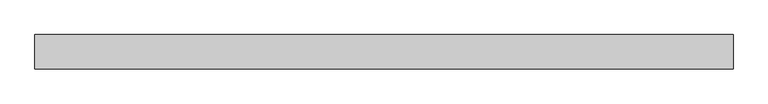
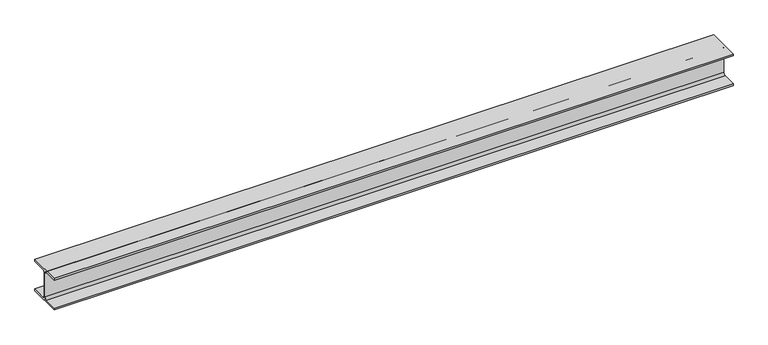
"""IFC4 building model written with IfcOpenShell, lengths in millimetres: beam geometry, 0912_Steel Framing_H-KSD3502 : H_SB_ASB_H-200x200x8x12."""

from ifc_helpers import new_model, si_unit, point, frame, frame_2d, origin, place, context, project, spatial, polyline, circle_curve, trimmed, segment, composite_curve, outline, extrude, source, transform, mapped, element, save


def beam_d7917815(model_context):
    return source(origin(), model_context, "Body", "SweptSolid", [
        extrude(outline(composite_curve([segment(polyline([(100.0, -88.0), (100.0, -100.0), (-100.0, -100.0), (-100.0, -88.0), (-17.0, -88.0)]), True, "CONTINUOUS"), segment(trimmed(circle_curve(frame_2d((-17.0, -75.0)), 13.0), [point((-17.0, -88.0))], [point((-4.0, -75.0))], True, "CARTESIAN"), True, "CONTINUOUS"), segment(polyline([(-4.0, -75.0), (-4.0, 75.0)]), True, "CONTINUOUS"), segment(trimmed(circle_curve(frame_2d((-17.0, 75.0)), 13.0), [point((-4.0, 75.0))], [point((-17.0, 88.0))], True, "CARTESIAN"), True, "CONTINUOUS"), segment(polyline([(-17.0, 88.0), (-100.0, 88.0), (-100.0, 100.0), (100.0, 100.0), (100.0, 88.0), (17.0, 88.0)]), True, "CONTINUOUS"), segment(trimmed(circle_curve(frame_2d((17.0, 75.0)), 13.0), [point((17.0, 88.0))], [point((4.0, 75.0))], True, "CARTESIAN"), True, "CONTINUOUS"), segment(polyline([(4.0, 75.0), (4.0, -75.0)]), True, "CONTINUOUS"), segment(trimmed(circle_curve(frame_2d((17.0, -75.0)), 13.0), [point((4.0, -75.0))], [point((17.0, -88.0))], True, "CARTESIAN"), True, "CONTINUOUS"), segment(polyline([(17.0, -88.0), (100.0, -88.0)]), True, "CONTINUOUS")], self_intersect=False)), frame((-2035.0333333, 0.0, 0.0), z_axis=(1.0, 0.0, 0.0), x_axis=(0.0, 1.0, 0.0)), (0.0, 0.0, 1.0), 4070.0666667),
    ])


if __name__ == "__main__":
    model = new_model("IFC4")
    model_context = context("Model", 3, world=origin())
    ifc_project = project(units=[si_unit("LENGTHUNIT", "METRE", prefix="MILLI")], contexts=[model_context])
    site = spatial("IfcSite", under=ifc_project)
    building = spatial("IfcBuilding", under=site)
    placement = place(None, origin())
    beam_shape = beam_d7917815(model_context)
    element("IfcBeam", 1, ObjectType="0912_Steel Framing_H-KSD3502 : H_SB_ASB_H-200x200x8x12", at=placement, inside=building, context=model_context, shape_type="MappedRepresentation", body=[
        mapped(beam_shape, transform((0.0, 0.0, 0.0), x_axis=(1.0, 0.0, 0.0), y_axis=(0.0, 1.0, 0.0), z_axis=(0.0, 0.0, 1.0))),
    ])
    save(model, "model.ifc")

# Revit data of these elements
# Type "0912_Steel Framing_H-KSD3502 : H_SB_ASB_H-200x200x8x12"
#   H_WM Code_1 = "S01AA002-00001 | Main Steel Structure Fabrication Work | Shelter/Building | Medium Steel - Standard (90KG/M>Weight≥30KG/M) | Material: (   )"
#   H_WM Code_2 = "S03AA028-00001 | Main Steel Structure Erection Work | Shelter/Building | Medium Steel (90KG/M>Weight≥30KG/M) | Material: (   )"
#   H_WM Code_3 = "S01AA010-00001 | Main Steel Structure Fabrication Work | Shelter/Building | Steel Painting/Coating | for Non-Fireproofed Steel Surface, Surface Preparation, Primer, Second & Final Coat | Material: (   )"
#   H_Q'ty Cal Type Tag = "SB-Q2"
#   Width = 20.0 cm
#   Web Thickness = 0.8 cm
#   Web Fillet = 1.3 cm
#   Warping Constant = 141000.0 cm⁶
#   W = 0
#   Torsional Moment of Inertia = 26.2485 cm⁴
#   Section Area = 63.53 cm²
#   Plastic Modulus weak axis = 244.0 cm³
#   Plastic Modulus strong axis = 525.0 cm³
#   Perimeter = 1.16 m²/m
#   Nominal Weight = 49.90 kgf/m
#   Moment of Inertia weak axis = 1600.00 cm⁴
#   Moment of Inertia strong axis = 4720.00 cm⁴
#   Height = 20.0 cm
#   Flange Thickness = 1.2 cm
#   Elastic Modulus weak axis = 160.0 cm³
#   Elastic Modulus strong axis = 472.0 cm³
#   Centroid Vertical = 10.0 cm
#   Centroid Horizontal = 10.0 cm
#   Ix = 47200000
#   Length [instance default] = 1.5240 m
#   Zx = 525000
#   b = 0.2000 m
#   h = 0.2000 m
#   r = 0.0130 m
#   s = 0.0080 m
#   t = 0.0120 m
#   A = 0.006353 m²
#   Structural Material [instance default] = Steel, 45-345
#   Assembly Code = ""
# Element 1 (IfcBeam, "0912_Steel Framing_H-KSD3502 : H_SB_ASB_H-200x200x8x12")
#   Structural Material = none
# Materials
#   "Steel, 45-345": class "Metal", colour RGB 189 187 185, transparency 0, Description = "Steel 345 MPa", Cost = 0
